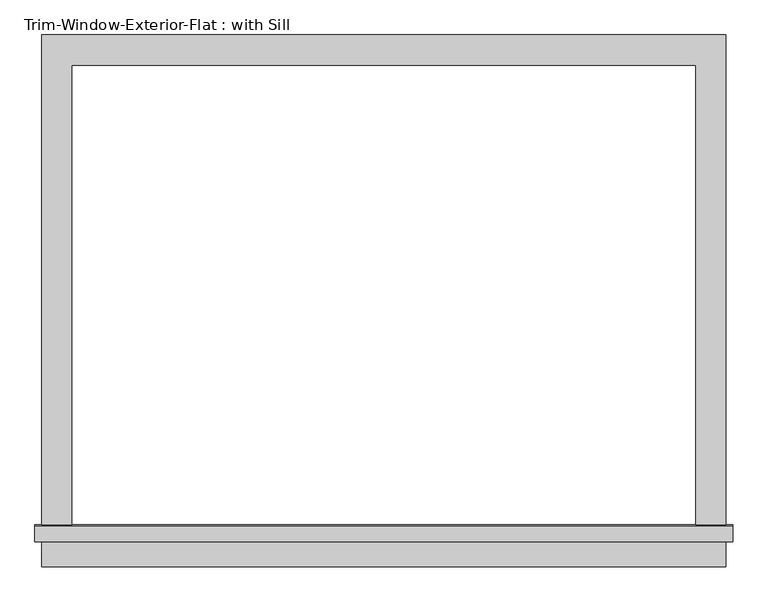
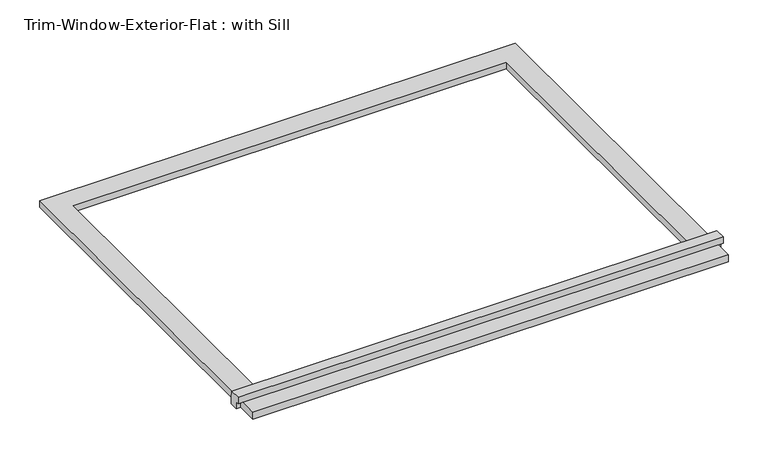
"""IFC4 building model written with IfcOpenShell, lengths in millimetres: proxy geometry, Trim-Window-Exterior-Flat : with Sill."""

import ifcopenshell
import ifcopenshell.guid

model = None  # the IFC model being written
_history = None  # IfcOwnerHistory: only IFC2X3 demands one
_inside = {}  # id of a spatial element -> (the spatial element, [elements in it])
_under = {}  # id of a project, library or spatial element -> (it, [spatial elements below it])
_declared = {}  # id of a project -> (the project, [libraries it declares])
_typed = {}  # id of a type object -> (the type object, [elements of that type])
_made_of = {}  # id of a material, layer set ... -> (it, [elements and type objects made of it])


def new_model(schema):
    """Start an empty IFC model of exactly this schema.

    Asked for "IFC4X3", IfcOpenShell would pick the latest addendum, in which some entities
    have other attributes; the version numbers below select the first issue.
    IFC2X3 requires an IfcOwnerHistory on every rooted entity: one is made here for all.
    """
    global model, _history
    if schema == "IFC4X3":
        model = ifcopenshell.file(schema_version=(4, 3, 0, 0))
    else:
        model = ifcopenshell.file(schema=schema)
    _inside.clear()
    _under.clear()
    _declared.clear()
    _typed.clear()
    _made_of.clear()
    _history = None
    if model.schema == "IFC2X3":
        org = make("IfcOrganization", Name="unknown")
        user = make(
            "IfcPersonAndOrganization",
            ThePerson=make("IfcPerson", FamilyName="unknown"),
            TheOrganization=org,
        )
        app = make(
            "IfcApplication",
            ApplicationDeveloper=org,
            Version="unknown",
            ApplicationFullName="unknown",
            ApplicationIdentifier="unknown",
        )
        _history = make(
            "IfcOwnerHistory",
            OwningUser=user,
            OwningApplication=app,
            ChangeAction="ADDED",
            CreationDate=0,
        )
    return model


def make(cls, **values):
    """One entity of the class cls with the attributes given. An attribute that is None is left unset."""
    return model.create_entity(
        cls, **{name: value for name, value in values.items() if value is not None}
    )


def rooted(cls, **values):
    """An entity with a GlobalId (a new one), such as an element, a storey or a relation."""
    return make(cls, GlobalId=ifcopenshell.guid.new(), OwnerHistory=_history, **values)


def si_unit(unit_type, name, prefix=None):
    """IfcSIUnit, for example si_unit("LENGTHUNIT", "METRE", prefix="MILLI")."""
    return make("IfcSIUnit", UnitType=unit_type, Prefix=prefix, Name=name)


def assignment(units):
    """IfcUnitAssignment: the units of a project."""
    return None if units is None else make("IfcUnitAssignment", Units=units)


def point(xyz):
    """IfcCartesianPoint."""
    return None if xyz is None else make("IfcCartesianPoint", Coordinates=xyz)


def direction(xyz):
    """IfcDirection."""
    return None if xyz is None else make("IfcDirection", DirectionRatios=xyz)


def frame(location, z_axis=None, x_axis=None):
    """IfcAxis2Placement3D, a coordinate frame: its origin and axes. An axis left out is left unset."""
    return make(
        "IfcAxis2Placement3D",
        Location=point(location),
        Axis=direction(z_axis),
        RefDirection=direction(x_axis),
    )


def origin():
    """The frame at (0, 0, 0) with its axes left unset."""
    return frame((0.0, 0.0, 0.0))


def origin_with_axes():
    """The frame at (0, 0, 0) with the z axis (0, 0, 1) and the x axis (1, 0, 0) written out."""
    return frame((0.0, 0.0, 0.0), z_axis=(0.0, 0.0, 1.0), x_axis=(1.0, 0.0, 0.0))


def place(relative_to, where):
    """IfcLocalPlacement: puts the frame where relative to a parent placement (None: the world)."""
    return make(
        "IfcLocalPlacement", PlacementRelTo=relative_to, RelativePlacement=where
    )


def context(
    kind, dimensions, precision=None, world=None, true_north=None, identifier=None
):
    """IfcGeometricRepresentationContext, for example the 3D "Model" context."""
    return make(
        "IfcGeometricRepresentationContext",
        ContextIdentifier=identifier,
        ContextType=kind,
        CoordinateSpaceDimension=dimensions,
        Precision=precision,
        WorldCoordinateSystem=world,
        TrueNorth=true_north,
    )


def project(units=None, contexts=None):
    """IfcProject with its units and contexts."""
    return rooted(
        "IfcProject",
        Name="project",
        RepresentationContexts=contexts,
        UnitsInContext=assignment(units),
    )


def spatial(cls, under=None, at=None, **own):
    """A site, building, storey or space (cls), placed at a placement, below another one or the project."""
    s = rooted(cls, ObjectPlacement=at, **own)
    if under is not None:
        _under.setdefault(under.id(), (under, []))[1].append(s)
    return s


def polyline(points):
    """IfcPolyline through the points."""
    return make("IfcPolyline", Points=[point(p) for p in points])


def outline(outer, holes=None, kind="AREA"):
    """IfcArbitraryClosedProfileDef: a profile drawn as a closed curve; with holes, ...WithVoids."""
    if holes is None:
        return make("IfcArbitraryClosedProfileDef", ProfileType=kind, OuterCurve=outer)
    return make(
        "IfcArbitraryProfileDefWithVoids",
        ProfileType=kind,
        OuterCurve=outer,
        InnerCurves=holes,
    )


def extrude(swept, where, along, depth):
    """IfcExtrudedAreaSolid: the profile swept, set in the frame where, extruded along a direction by depth."""
    return make(
        "IfcExtrudedAreaSolid",
        SweptArea=swept,
        Position=where,
        ExtrudedDirection=direction(along),
        Depth=depth,
    )


def shape(context_of_items, identifier, shape_type, items):
    """IfcShapeRepresentation: the items that make up one representation, for example the "Body"."""
    return make(
        "IfcShapeRepresentation",
        ContextOfItems=context_of_items,
        RepresentationIdentifier=identifier,
        RepresentationType=shape_type,
        Items=items,
    )


def source(mapping_origin, context_of_items, identifier, shape_type, items):
    """IfcRepresentationMap: a shape defined once, which mapped items show again and again."""
    return make(
        "IfcRepresentationMap",
        MappingOrigin=mapping_origin,
        MappedRepresentation=shape(context_of_items, identifier, shape_type, items),
    )


def transform(
    local_origin,
    x_axis=None,
    y_axis=None,
    z_axis=None,
    scale=None,
    scale2=None,
    scale3=None,
    uniform=True,
):
    """IfcCartesianTransformationOperator3D, or its non-uniform kind. x_axis, y_axis, z_axis: its Axis1, 2, 3."""
    if uniform:
        return make(
            "IfcCartesianTransformationOperator3D",
            Axis1=direction(x_axis),
            Axis2=direction(y_axis),
            LocalOrigin=point(local_origin),
            Scale=scale,
            Axis3=direction(z_axis),
        )
    return make(
        "IfcCartesianTransformationOperator3DnonUniform",
        Axis1=direction(x_axis),
        Axis2=direction(y_axis),
        LocalOrigin=point(local_origin),
        Scale=scale,
        Axis3=direction(z_axis),
        Scale2=scale2,
        Scale3=scale3,
    )


def mapped(mapping_source, mapping_target):
    """IfcMappedItem: shows the shape of a source again, moved by a transform."""
    return make(
        "IfcMappedItem", MappingSource=mapping_source, MappingTarget=mapping_target
    )


def made_of(thing, what):
    """Note that an element or type object is made of a material, layer set ...; save() writes the relation."""
    if what is not None:
        _made_of.setdefault(what.id(), (what, []))[1].append(thing)
    return thing


def element(
    cls,
    number,
    at=None,
    inside=None,
    cuts=None,
    type_object=None,
    material=None,
    context=None,
    identifier="Body",
    shape_type=None,
    held_by="IfcProductDefinitionShape",
    body=None,
    shapes=None,
    **own,
):
    """One element of the class cls, such as IfcWall. Its Tag is "e" and its number.

    at: its placement. inside: the storey or other place that contains it. cuts: it is an
    opening in that element (IfcRelVoidsElement). A single representation is given by context,
    identifier, shape_type and body (its items); several are given by shapes. held_by: the class
    of the entity that holds the representations. save() writes the other relations.
    """
    e = rooted(cls, Tag="e%d" % number, ObjectPlacement=at, **own)
    if body is not None:
        shapes = [shape(context, identifier, shape_type, body)]
    if shapes is not None:
        e.Representation = make(held_by, Representations=shapes)
    if inside is not None:
        _inside.setdefault(inside.id(), (inside, []))[1].append(e)
    if cuts is not None:
        rooted(
            "IfcRelVoidsElement", RelatingBuildingElement=cuts, RelatedOpeningElement=e
        )
    if type_object is not None:
        _typed.setdefault(type_object.id(), (type_object, []))[1].append(e)
    return made_of(e, material)


def aggregate(whole, parts):
    """IfcRelAggregates: a whole, such as a stair, and the parts it consists of."""
    return rooted("IfcRelAggregates", RelatingObject=whole, RelatedObjects=parts)


def save(model, path):
    """Write the relations noted so far, then the file.

    IfcRelAggregates (storeys below a building ...), IfcRelContainedInSpatialStructure (elements
    in a storey), IfcRelDefinesByType, IfcRelAssociatesMaterial and IfcRelDeclares: one each for
    every whole, place, type object, material and project.
    """
    for whole, parts in _under.values():
        aggregate(whole, parts)
    for where, things in _inside.values():
        rooted(
            "IfcRelContainedInSpatialStructure",
            RelatedElements=things,
            RelatingStructure=where,
        )
    for kind, things in _typed.values():
        rooted("IfcRelDefinesByType", RelatedObjects=things, RelatingType=kind)
    for what, things in _made_of.values():
        rooted("IfcRelAssociatesMaterial", RelatedObjects=things, RelatingMaterial=what)
    for by, libraries in _declared.values():
        rooted("IfcRelDeclares", RelatingContext=by, RelatedDefinitions=libraries)
    model.write(path)


def trim_window_exterior_flat_with_sill_a6ca139b(model_context):
    return source(origin(), model_context, "Body", "SweptSolid", [
        extrude(outline(polyline([(647.7, -892.1323709), (647.7, -949.2823709), (-647.7, -949.2823709), (-647.7, -892.1323709), (647.7, -892.1323709)])), origin_with_axes(), (0.0, 0.0, 1.0), 19.05),
        extrude(outline(polyline([(-901.7, 38.1), (-872.4080645, 38.1), (-869.95, 19.05), (-869.95, 0.0), (-892.1323709, 0.0), (-892.1323709, 19.05), (-901.7, 19.05), (-901.7, 38.1)])), frame((-660.4, 0.0, 0.0), z_axis=(1.0, 0.0, 0.0), x_axis=(0.0, 1.0, 0.0)), (0.0, 0.0, 1.0), 1320.8),
        extrude(outline(polyline([(-647.7, 57.15), (647.7, 57.15), (647.7, -869.95), (590.55, -869.95), (590.55, 0.0), (-590.55, 0.0), (-590.55, -869.95), (-647.7, -869.95), (-647.7, 57.15)])), origin_with_axes(), (0.0, 0.0, 1.0), 19.05),
    ])


if __name__ == "__main__":
    model = new_model("IFC4")
    model_context = context("Model", 3, world=origin())
    ifc_project = project(units=[si_unit("LENGTHUNIT", "METRE", prefix="MILLI")], contexts=[model_context])
    site = spatial("IfcSite", under=ifc_project)
    building = spatial("IfcBuilding", under=site)
    placement = place(None, origin())
    trim_window_exterior_flat_with_sill_shape = trim_window_exterior_flat_with_sill_a6ca139b(model_context)
    element("IfcBuildingElementProxy", 1, Name="Trim-Window-Exterior-Flat : with Sill", ObjectType="Trim-Window-Exterior-Flat : with Sill", at=placement, inside=building, context=model_context, shape_type="MappedRepresentation", body=[
        mapped(trim_window_exterior_flat_with_sill_shape, transform((0.0, 0.0, 0.0), x_axis=(1.0, 0.0, 0.0), y_axis=(0.0, 1.0, 0.0), z_axis=(0.0, 0.0, 1.0))),
    ])
    save(model, "model.ifc")

# Revit data of these elements
# Type "Trim-Window-Exterior-Flat : with Sill"
#   Trim Width = 0' - 2 1/4"
#   Trim Thickness_Picture Frame = 0' - 1 1/4"
#   Trim Thickness_with Sill = 0' - 0 3/4"
#   Sill Thickness = 0' - 1 1/4"
#   Opening Width [instance default] = 2' - 0"
#   Opening Height [instance default] = 3' - 0"
#   Default Elevation = 4' - 0"
#   Sill = yes
#   Picture Frame = no
#   Trim Material [instance default] = none
# Element 1 (IfcBuildingElementProxy, "Trim-Window-Exterior-Flat : with Sill")
#   Opening Width = 3' - 10 1/2"
#   Opening Height = 2' - 10 1/4"
#   Trim Material = Clad - White
#   Materials on its faces: "Clad - White"
# Materials
#   "Clad - White": class "Wood", colour RGB 242 242 238, transparency 0, Cost = 0
